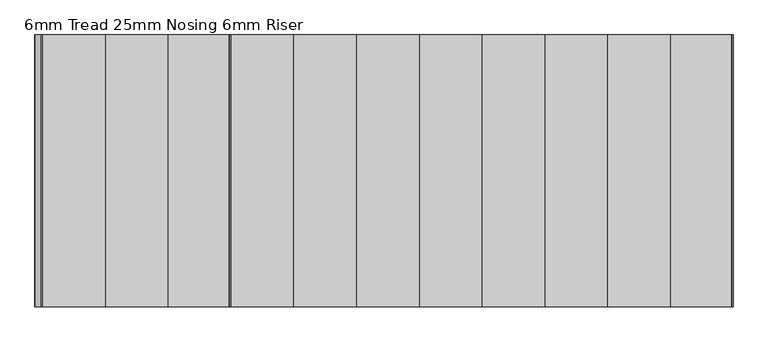
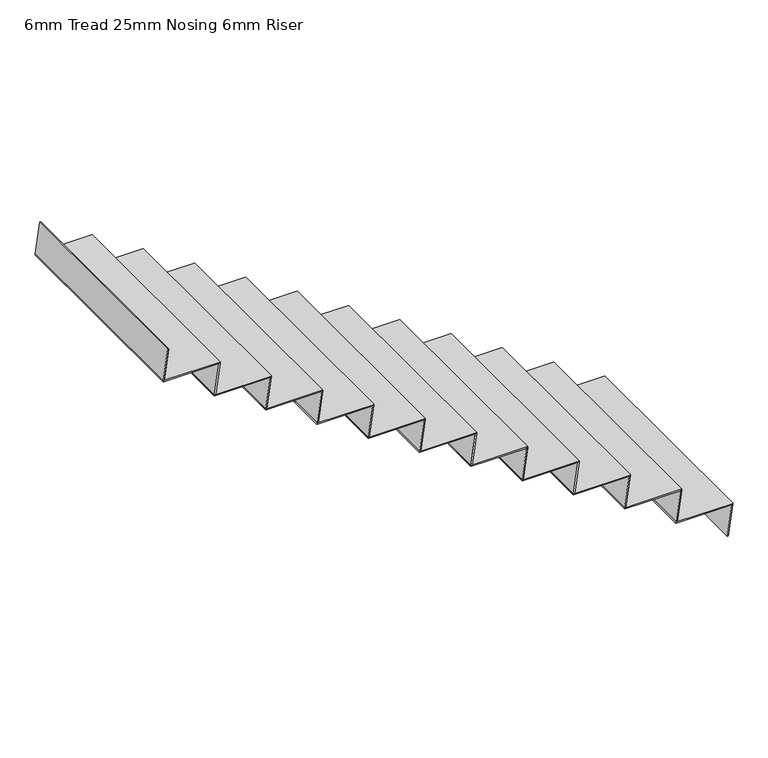
"""IFC4 building model written with IfcOpenShell, lengths in millimetres: stair flight geometry, 6mm Tread 25mm Nosing 6mm Riser."""

from ifc_helpers import new_model, si_unit, frame, origin, place, context, project, spatial, polyline, outline, extrude, source, transform, mapped, element, save


def stair_flight_6mm_tread_25mm_nosing_6mm_riser_ac762ffa(model_context):
    return source(origin(), model_context, "Body", "SweptSolid", [
        extrude(outline(polyline([(26529.4117647, 16350.0), (26529.4117647, 16043.9400908), (26523.4117647, 16043.0900908), (26523.4117647, 16349.15), (26529.4117647, 16350.0)])), frame((0.0, 12030.4345331, 0.0), z_axis=(0.0, 1.0, 0.0), x_axis=(0.0, 0.0, 1.0)), (0.0, 0.0, 1.0), 1190.0),
        extrude(outline(polyline([(26523.4117647, 16349.15), (26523.4117647, 16343.0900908), (26352.9411765, 16318.9400908), (26352.9411765, 16325.0), (26523.4117647, 16349.15)])), frame((0.0, 12030.4345331, 0.0), z_axis=(0.0, 1.0, 0.0), x_axis=(0.0, 0.0, 1.0)), (0.0, 0.0, 1.0), 1190.0),
        extrude(outline(polyline([(26699.8823529, 16074.15), (26699.8823529, 16068.0900908), (26529.4117647, 16043.9400908), (26529.4117647, 16050.0), (26699.8823529, 16074.15)])), frame((0.0, 12030.4345331, 0.0), z_axis=(0.0, 1.0, 0.0), x_axis=(0.0, 0.0, 1.0)), (0.0, 0.0, 1.0), 1190.0),
        extrude(outline(polyline([(26705.8823529, 16075.0), (26705.8823529, 15768.9400908), (26699.8823529, 15768.0900908), (26699.8823529, 16074.15), (26705.8823529, 16075.0)])), frame((0.0, 12030.4345331, 0.0), z_axis=(0.0, 1.0, 0.0), x_axis=(0.0, 0.0, 1.0)), (0.0, 0.0, 1.0), 1190.0),
        extrude(outline(polyline([(26876.3529412, 15799.15), (26876.3529412, 15793.0900908), (26705.8823529, 15768.9400908), (26705.8823529, 15775.0), (26876.3529412, 15799.15)])), frame((0.0, 12030.4345331, 0.0), z_axis=(0.0, 1.0, 0.0), x_axis=(0.0, 0.0, 1.0)), (0.0, 0.0, 1.0), 1190.0),
        extrude(outline(polyline([(26882.3529412, 15800.0), (26882.3529412, 15493.9400908), (26876.3529412, 15493.0900908), (26876.3529412, 15799.15), (26882.3529412, 15800.0)])), frame((0.0, 12030.4345331, 0.0), z_axis=(0.0, 1.0, 0.0), x_axis=(0.0, 0.0, 1.0)), (0.0, 0.0, 1.0), 1190.0),
        extrude(outline(polyline([(27052.8235294, 15524.15), (27052.8235294, 15518.0900908), (26882.3529412, 15493.9400908), (26882.3529412, 15500.0), (27052.8235294, 15524.15)])), frame((0.0, 12030.4345331, 0.0), z_axis=(0.0, 1.0, 0.0), x_axis=(0.0, 0.0, 1.0)), (0.0, 0.0, 1.0), 1190.0),
        extrude(outline(polyline([(27058.8235294, 15525.0), (27058.8235294, 15218.9400908), (27052.8235294, 15218.0900908), (27052.8235294, 15524.15), (27058.8235294, 15525.0)])), frame((0.0, 12030.4345331, 0.0), z_axis=(0.0, 1.0, 0.0), x_axis=(0.0, 0.0, 1.0)), (0.0, 0.0, 1.0), 1190.0),
        extrude(outline(polyline([(27229.2941176, 15249.15), (27229.2941176, 15243.0900908), (27058.8235294, 15218.9400908), (27058.8235294, 15225.0), (27229.2941176, 15249.15)])), frame((0.0, 12030.4345331, 0.0), z_axis=(0.0, 1.0, 0.0), x_axis=(0.0, 0.0, 1.0)), (0.0, 0.0, 1.0), 1190.0),
        extrude(outline(polyline([(27235.2941176, 15250.0), (27235.2941176, 14943.9400908), (27229.2941176, 14943.0900908), (27229.2941176, 15249.15), (27235.2941176, 15250.0)])), frame((0.0, 12030.4345331, 0.0), z_axis=(0.0, 1.0, 0.0), x_axis=(0.0, 0.0, 1.0)), (0.0, 0.0, 1.0), 1190.0),
        extrude(outline(polyline([(27405.7647059, 14974.15), (27405.7647059, 14968.0900908), (27235.2941176, 14943.9400908), (27235.2941176, 14950.0), (27405.7647059, 14974.15)])), frame((0.0, 12030.4345331, 0.0), z_axis=(0.0, 1.0, 0.0), x_axis=(0.0, 0.0, 1.0)), (0.0, 0.0, 1.0), 1190.0),
        extrude(outline(polyline([(27411.7647059, 14975.0), (27411.7647059, 14668.9400908), (27405.7647059, 14668.0900908), (27405.7647059, 14974.15), (27411.7647059, 14975.0)])), frame((0.0, 12030.4345331, 0.0), z_axis=(0.0, 1.0, 0.0), x_axis=(0.0, 0.0, 1.0)), (0.0, 0.0, 1.0), 1190.0),
        extrude(outline(polyline([(27582.2352941, 14699.15), (27582.2352941, 14693.0900908), (27411.7647059, 14668.9400908), (27411.7647059, 14675.0), (27582.2352941, 14699.15)])), frame((0.0, 12030.4345331, 0.0), z_axis=(0.0, 1.0, 0.0), x_axis=(0.0, 0.0, 1.0)), (0.0, 0.0, 1.0), 1190.0),
        extrude(outline(polyline([(27588.2352941, 14700.0), (27588.2352941, 14393.9400908), (27582.2352941, 14393.0900908), (27582.2352941, 14699.15), (27588.2352941, 14700.0)])), frame((0.0, 12030.4345331, 0.0), z_axis=(0.0, 1.0, 0.0), x_axis=(0.0, 0.0, 1.0)), (0.0, 0.0, 1.0), 1190.0),
        extrude(outline(polyline([(27758.7058824, 14424.15), (27758.7058824, 14418.0900908), (27588.2352941, 14393.9400908), (27588.2352941, 14400.0), (27758.7058824, 14424.15)])), frame((0.0, 12030.4345331, 0.0), z_axis=(0.0, 1.0, 0.0), x_axis=(0.0, 0.0, 1.0)), (0.0, 0.0, 1.0), 1190.0),
        extrude(outline(polyline([(27764.7058824, 14425.0), (27764.7058824, 14118.9400908), (27758.7058824, 14118.0900908), (27758.7058824, 14424.15), (27764.7058824, 14425.0)])), frame((0.0, 12030.4345331, 0.0), z_axis=(0.0, 1.0, 0.0), x_axis=(0.0, 0.0, 1.0)), (0.0, 0.0, 1.0), 1190.0),
        extrude(outline(polyline([(27935.1764706, 14149.15), (27935.1764706, 14143.0900908), (27764.7058824, 14118.9400908), (27764.7058824, 14125.0), (27935.1764706, 14149.15)])), frame((0.0, 12030.4345331, 0.0), z_axis=(0.0, 1.0, 0.0), x_axis=(0.0, 0.0, 1.0)), (0.0, 0.0, 1.0), 1190.0),
        extrude(outline(polyline([(27941.1764706, 14150.0), (27941.1764706, 13843.9400908), (27935.1764706, 13843.0900908), (27935.1764706, 14149.15), (27941.1764706, 14150.0)])), frame((0.0, 12030.4345331, 0.0), z_axis=(0.0, 1.0, 0.0), x_axis=(0.0, 0.0, 1.0)), (0.0, 0.0, 1.0), 1190.0),
        extrude(outline(polyline([(28111.6470588, 13874.15), (28111.6470588, 13868.0900908), (27941.1764706, 13843.9400908), (27941.1764706, 13850.0), (28111.6470588, 13874.15)])), frame((0.0, 12030.4345331, 0.0), z_axis=(0.0, 1.0, 0.0), x_axis=(0.0, 0.0, 1.0)), (0.0, 0.0, 1.0), 1190.0),
        extrude(outline(polyline([(28117.6470588, 13875.0), (28117.6470588, 13568.9400908), (28111.6470588, 13568.0900908), (28111.6470588, 13874.15), (28117.6470588, 13875.0)])), frame((0.0, 12030.4345331, 0.0), z_axis=(0.0, 1.0, 0.0), x_axis=(0.0, 0.0, 1.0)), (0.0, 0.0, 1.0), 1190.0),
        extrude(outline(polyline([(28288.1176471, 13599.15), (28288.1176471, 13593.0900908), (28117.6470588, 13568.9400908), (28117.6470588, 13575.0), (28288.1176471, 13599.15)])), frame((0.0, 12030.4345331, 0.0), z_axis=(0.0, 1.0, 0.0), x_axis=(0.0, 0.0, 1.0)), (0.0, 0.0, 1.0), 1190.0),
        extrude(outline(polyline([(28464.5882353, 13324.15), (28464.5882353, 13318.0900908), (28294.1176471, 13293.9400908), (28294.1176471, 13300.0), (28464.5882353, 13324.15)])), frame((0.0, 12030.4345331, 0.0), z_axis=(0.0, 1.0, 0.0), x_axis=(0.0, 0.0, 1.0)), (0.0, 0.0, 1.0), 1190.0),
        extrude(outline(polyline([(28294.1176471, 13600.0), (28294.1176471, 13293.9400908), (28288.1176471, 13293.0900908), (28288.1176471, 13599.15), (28294.1176471, 13600.0)])), frame((0.0, 12030.4345331, 0.0), z_axis=(0.0, 1.0, 0.0), x_axis=(0.0, 0.0, 1.0)), (0.0, 0.0, 1.0), 1190.0),
    ])


if __name__ == "__main__":
    model = new_model("IFC4")
    model_context = context("Model", 3, world=origin())
    ifc_project = project(units=[si_unit("LENGTHUNIT", "METRE", prefix="MILLI")], contexts=[model_context])
    site = spatial("IfcSite", under=ifc_project)
    building = spatial("IfcBuilding", under=site)
    placement = place(None, origin())
    stair_flight_6mm_tread_25mm_nosing_6mm_riser_shape = stair_flight_6mm_tread_25mm_nosing_6mm_riser_ac762ffa(model_context)
    element("IfcStairFlight", 1, ObjectType="6mm Tread 25mm Nosing 6mm Riser", at=placement, inside=building, context=model_context, shape_type="MappedRepresentation", body=[
        mapped(stair_flight_6mm_tread_25mm_nosing_6mm_riser_shape, transform((0.0, 0.0, 0.0), x_axis=(1.0, 0.0, 0.0), y_axis=(0.0, 1.0, 0.0), z_axis=(0.0, 0.0, 1.0))),
    ])
    save(model, "model.ifc")

# Revit data of these elements
# Element 1 (IfcStairFlight, "6mm Tread 25mm Nosing 6mm Riser")
#   Materials on its faces: "Steel, Paint Finish, Dark Gray"
# Materials
#   "Steel, Paint Finish, Dark Gray": class "Metal", colour RGB 89 89 89, transparency 0, Description = "Steel, paint finish, dark gray, glossy", Cost = 0
